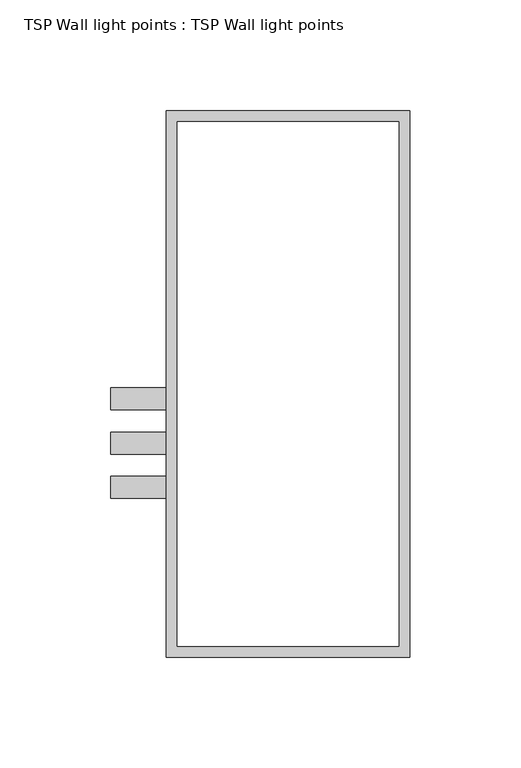
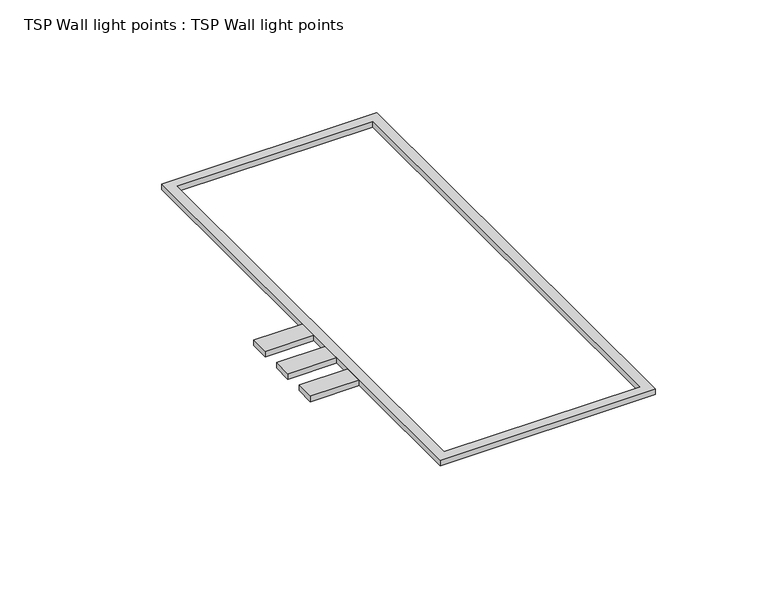
"""IFC4 building model written with IfcOpenShell, lengths in millimetres: proxy geometry, TSP Wall light points : TSP Wall light points."""

from ifc_helpers import new_model, si_unit, origin, origin_with_axes, place, context, project, spatial, polyline, outline, extrude, source, transform, mapped, element, save


def tsp_wall_light_points_tsp_wall_light_points_45c911df(model_context):
    return source(origin(), model_context, "Body", "SweptSolid", [
        extrude(outline(polyline([(105.0, 125.0229032), (105.0, -121.6770968), (-5.0, -121.6770968), (-5.0, 125.0229032), (105.0, 125.0229032)]), holes=[polyline([(100.0, 120.0229032), (0.0, 120.0229032), (0.0, -116.6770968), (100.0, -116.6770968), (100.0, 120.0229032)])]), origin_with_axes(), (0.0, 0.0, 1.0), 3.0),
        extrude(outline(polyline([(-30.0, 0.0), (-5.0, 0.0), (-5.0, -10.0), (-30.0, -10.0), (-30.0, 0.0)])), origin_with_axes(), (0.0, 0.0, 1.0), 3.0),
        extrude(outline(polyline([(-30.0, -20.0), (-5.0, -20.0), (-5.0, -30.0), (-30.0, -30.0), (-30.0, -20.0)])), origin_with_axes(), (0.0, 0.0, 1.0), 3.0),
        extrude(outline(polyline([(-30.0, -40.0), (-5.0, -40.0), (-5.0, -50.0), (-30.0, -50.0), (-30.0, -40.0)])), origin_with_axes(), (0.0, 0.0, 1.0), 3.0),
    ])


if __name__ == "__main__":
    model = new_model("IFC4")
    model_context = context("Model", 3, world=origin())
    ifc_project = project(units=[si_unit("LENGTHUNIT", "METRE", prefix="MILLI")], contexts=[model_context])
    site = spatial("IfcSite", under=ifc_project)
    building = spatial("IfcBuilding", under=site)
    placement = place(None, origin())
    tsp_wall_light_points_tsp_wall_light_points_shape = tsp_wall_light_points_tsp_wall_light_points_45c911df(model_context)
    element("IfcBuildingElementProxy", 1, Name="TSP Wall light points : TSP Wall light points", ObjectType="TSP Wall light points : TSP Wall light points", at=placement, inside=building, context=model_context, shape_type="MappedRepresentation", body=[
        mapped(tsp_wall_light_points_tsp_wall_light_points_shape, transform((0.0, 0.0, 0.0), x_axis=(1.0, 0.0, 0.0), y_axis=(0.0, 1.0, 0.0), z_axis=(0.0, 0.0, 1.0))),
    ])
    save(model, "model.ifc")

# Revit data of these elements
# Type "TSP Wall light points : TSP Wall light points"
#   Model = "TSP_ELEC220WLP"
#   Default Elevation = 0
# Element 1 (IfcBuildingElementProxy, "TSP Wall light points : TSP Wall light points")
#   Materials on its faces: "Plastic, Opaque Black"
# Materials
#   "Plastic, Opaque Black": class "Plastic", colour RGB 0 0 0, transparency 0.7, Description = "Plastic, generic, opaque black", Cost = 0
